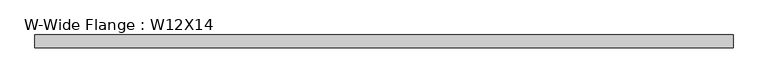
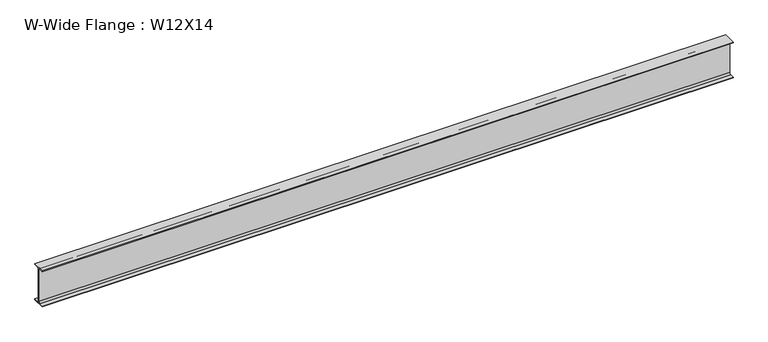
"""IFC4 building model written with IfcOpenShell, lengths in millimetres: beam geometry, W-Wide Flange : W12X14."""

from ifc_helpers import new_model, si_unit, point, frame, frame_2d, origin, place, context, project, spatial, polyline, circle_curve, trimmed, segment, composite_curve, outline, extrude, source, transform, mapped, element, save


def w_wide_flange_w12x14_7ace5727(model_context):
    return source(origin(), model_context, "Body", "SweptSolid", [
        extrude(outline(composite_curve([segment(polyline([(50.419, -145.415), (50.419, -151.13), (-50.419, -151.13), (-50.419, -145.415), (-15.875, -145.415)]), True, "CONTINUOUS"), segment(trimmed(circle_curve(frame_2d((-15.875, -132.08)), 13.335), [point((-15.875, -145.415))], [point((-2.54, -132.08))], True, "CARTESIAN"), True, "CONTINUOUS"), segment(polyline([(-2.54, -132.08), (-2.54, 132.08)]), True, "CONTINUOUS"), segment(trimmed(circle_curve(frame_2d((-15.875, 132.08)), 13.335), [point((-2.54, 132.08))], [point((-15.875, 145.415))], True, "CARTESIAN"), True, "CONTINUOUS"), segment(polyline([(-15.875, 145.415), (-50.419, 145.415), (-50.419, 151.13), (50.419, 151.13), (50.419, 145.415), (15.875, 145.415)]), True, "CONTINUOUS"), segment(trimmed(circle_curve(frame_2d((15.875, 132.08)), 13.335), [point((15.875, 145.415))], [point((2.54, 132.08))], True, "CARTESIAN"), True, "CONTINUOUS"), segment(polyline([(2.54, 132.08), (2.54, -132.08)]), True, "CONTINUOUS"), segment(trimmed(circle_curve(frame_2d((15.875, -132.08)), 13.335), [point((2.54, -132.08))], [point((15.875, -145.415))], True, "CARTESIAN"), True, "CONTINUOUS"), segment(polyline([(15.875, -145.415), (50.419, -145.415)]), True, "CONTINUOUS")], self_intersect=False)), frame((-2755.9, 0.0, 0.0), z_axis=(1.0, 0.0, 0.0), x_axis=(0.0, 1.0, 0.0)), (0.0, 0.0, 1.0), 5511.8),
    ])


if __name__ == "__main__":
    model = new_model("IFC4")
    model_context = context("Model", 3, world=origin())
    ifc_project = project(units=[si_unit("LENGTHUNIT", "METRE", prefix="MILLI")], contexts=[model_context])
    site = spatial("IfcSite", under=ifc_project)
    building = spatial("IfcBuilding", under=site)
    placement = place(None, origin())
    w_wide_flange_w12x14_shape = w_wide_flange_w12x14_7ace5727(model_context)
    element("IfcBeam", 1, ObjectType="W-Wide Flange : W12X14", at=placement, inside=building, context=model_context, shape_type="MappedRepresentation", body=[
        mapped(w_wide_flange_w12x14_shape, transform((0.0, 0.0, 0.0), x_axis=(1.0, 0.0, 0.0), y_axis=(0.0, 1.0, 0.0), z_axis=(0.0, 0.0, 1.0))),
    ])
    save(model, "model.ifc")

# Revit data of these elements
# Type "W-Wide Flange : W12X14"
#   Assembly Code = "B10"
#   W = 14
#   Length [instance default] = 5' - 0"
#   bf = 0' - 3.97"
#   d = 0' - 11.9"
#   k = 0' - 0 3/4"
#   k2 = 0' - 0.525"
#   tf = 0' - 0.225"
#   tw = 0' - 0.2"
#   A = 0.0288889 SF
#   Structural Material [instance default] = Steel ASTM A992
# Element 1 (IfcBeam, "W-Wide Flange : W12X14")
#   Materials on its faces: "Steel ASTM A992"
# Materials
#   "Steel ASTM A992": class "Metal", colour RGB 199 199 199, transparency 0, Description = "Structural steel 50ksi", Cost = 0
